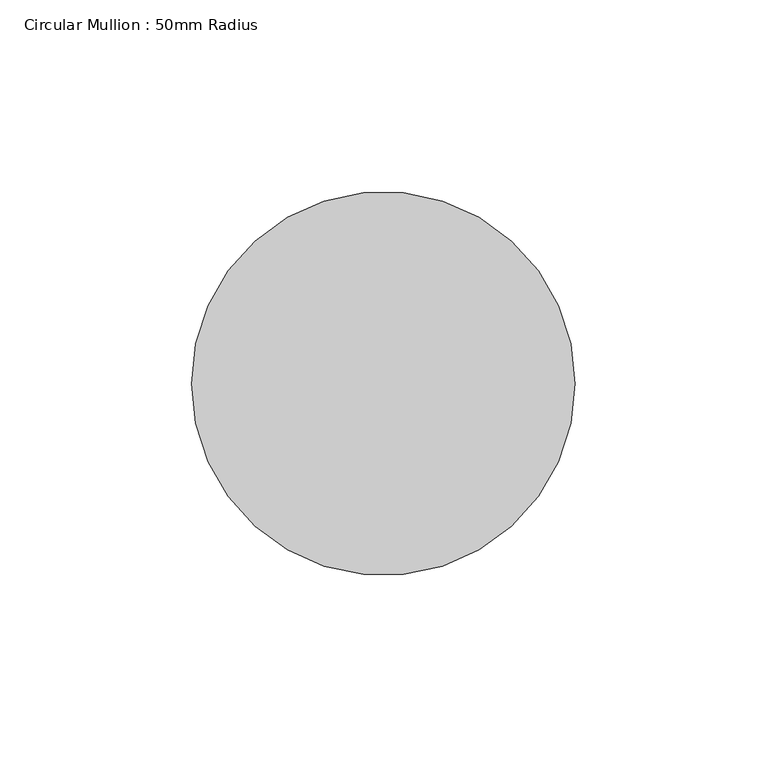
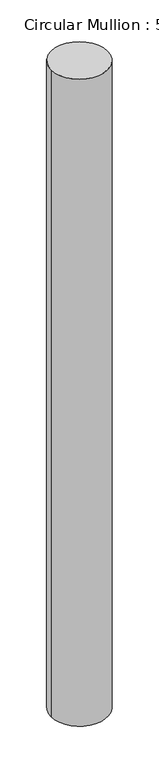
"""IFC4 building model written with IfcOpenShell, lengths in millimetres: member geometry, Circular Mullion : 50mm Radius."""

from ifc_helpers import new_model, si_unit, point, frame, origin, origin_2d, place, context, project, spatial, circle_curve, trimmed, segment, composite_curve, outline, extrude, source, transform, mapped, element, save


def circular_mullion_50mm_radius_82d39af2(model_context):
    return source(origin(), model_context, "Body", "SweptSolid", [
        extrude(outline(composite_curve([segment(trimmed(circle_curve(origin_2d(), 50.0), [point((50.0, 0.0))], [point((-50.0, 0.0))], False, "CARTESIAN"), True, "CONTINUOUS"), segment(trimmed(circle_curve(origin_2d(), 50.0), [point((-50.0, 0.0))], [point((50.0, 0.0))], False, "CARTESIAN"), True, "CONTINUOUS")], self_intersect=False)), frame((0.0, 0.0, -1208.8143283), z_axis=(0.0, 0.0, 1.0), x_axis=(1.0, 0.0, 0.0)), (0.0, 0.0, 1.0), 1208.8143283),
    ])


if __name__ == "__main__":
    model = new_model("IFC4")
    model_context = context("Model", 3, world=origin())
    ifc_project = project(units=[si_unit("LENGTHUNIT", "METRE", prefix="MILLI")], contexts=[model_context])
    site = spatial("IfcSite", under=ifc_project)
    building = spatial("IfcBuilding", under=site)
    placement = place(None, origin())
    circular_mullion_50mm_radius_shape = circular_mullion_50mm_radius_82d39af2(model_context)
    element("IfcMember", 1, ObjectType="Circular Mullion : 50mm Radius", at=placement, inside=building, context=model_context, shape_type="MappedRepresentation", body=[
        mapped(circular_mullion_50mm_radius_shape, transform((0.0, 0.0, 0.0), x_axis=(1.0, 0.0, 0.0), y_axis=(0.0, 1.0, 0.0), z_axis=(0.0, 0.0, 1.0))),
    ])
    save(model, "model.ifc")

# Revit data of these elements
# Type "Circular Mullion : 50mm Radius"
#   built-in parameter 1007350 = 0.164042 (stored number, unit not read)
# Element 1 (IfcMember, "Circular Mullion : 50mm Radius")
#   Materials on its faces: "Aluminium"
# Materials
#   "Aluminium": class "Metal", colour RGB 247 247 247, transparency 0, Description = "Aluminium 6061", Cost = 0
